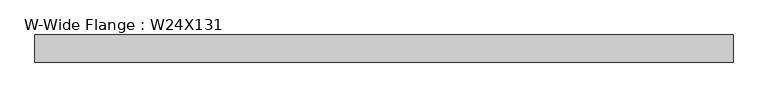
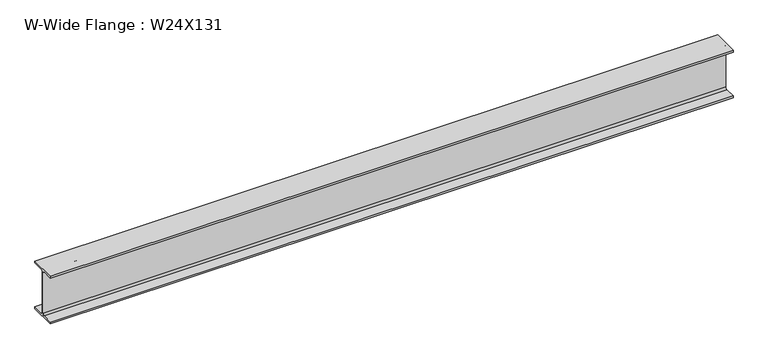
"""IFC4 building model written with IfcOpenShell, lengths in millimetres: beam geometry, W-Wide Flange : W24X131."""

from ifc_helpers import new_model, si_unit, point, frame, frame_2d, origin, place, context, project, spatial, polyline, circle_curve, trimmed, segment, composite_curve, outline, extrude, source, transform, mapped, element, save


def w_wide_flange_w24x131_18549e9f(model_context):
    return source(origin(), model_context, "Body", "SweptSolid", [
        extrude(outline(composite_curve([segment(polyline([(163.83, -286.766), (163.83, -311.15), (-163.83, -311.15), (-163.83, -286.766), (-30.9245, -286.766)]), True, "CONTINUOUS"), segment(trimmed(circle_curve(frame_2d((-30.9245, -263.525)), 23.241), [point((-30.9245, -286.766))], [point((-7.6835, -263.525))], True, "CARTESIAN"), True, "CONTINUOUS"), segment(polyline([(-7.6835, -263.525), (-7.6835, 263.525)]), True, "CONTINUOUS"), segment(trimmed(circle_curve(frame_2d((-30.9245, 263.525)), 23.241), [point((-7.6835, 263.525))], [point((-30.9245, 286.766))], True, "CARTESIAN"), True, "CONTINUOUS"), segment(polyline([(-30.9245, 286.766), (-163.83, 286.766), (-163.83, 311.15), (163.83, 311.15), (163.83, 286.766), (30.9245, 286.766)]), True, "CONTINUOUS"), segment(trimmed(circle_curve(frame_2d((30.9245, 263.525)), 23.241), [point((30.9245, 286.766))], [point((7.6835, 263.525))], True, "CARTESIAN"), True, "CONTINUOUS"), segment(polyline([(7.6835, 263.525), (7.6835, -263.525)]), True, "CONTINUOUS"), segment(trimmed(circle_curve(frame_2d((30.9245, -263.525)), 23.241), [point((7.6835, -263.525))], [point((30.9245, -286.766))], True, "CARTESIAN"), True, "CONTINUOUS"), segment(polyline([(30.9245, -286.766), (163.83, -286.766)]), True, "CONTINUOUS")], self_intersect=False)), frame((-4213.6230758, 0.0, 0.0), z_axis=(1.0, 0.0, 0.0), x_axis=(0.0, 1.0, 0.0)), (0.0, 0.0, 1.0), 8427.2461516),
    ])


if __name__ == "__main__":
    model = new_model("IFC4")
    model_context = context("Model", 3, world=origin())
    ifc_project = project(units=[si_unit("LENGTHUNIT", "METRE", prefix="MILLI")], contexts=[model_context])
    site = spatial("IfcSite", under=ifc_project)
    building = spatial("IfcBuilding", under=site)
    placement = place(None, origin())
    w_wide_flange_w24x131_shape = w_wide_flange_w24x131_18549e9f(model_context)
    element("IfcBeam", 1, ObjectType="W-Wide Flange : W24X131", at=placement, inside=building, context=model_context, shape_type="MappedRepresentation", body=[
        mapped(w_wide_flange_w24x131_shape, transform((0.0, 0.0, 0.0), x_axis=(1.0, 0.0, 0.0), y_axis=(0.0, 1.0, 0.0), z_axis=(0.0, 0.0, 1.0))),
    ])
    save(model, "model.ifc")

# Revit data of these elements
# Type "W-Wide Flange : W24X131"
#   Assembly Code = "B10"
#   W = 131
#   Start Extension Calculation [instance default] = 10' - 0"
#   Start Extension [instance default] = -0' - 0 1/2"
#   End Extension Calculation [instance default] = 10' - 0"
#   End Extension [instance default] = -0' - 0 1/2"
#   Length [instance default] = 5' - 0"
#   bf = 1' - 0.9"
#   d = 2' - 0 1/2"
#   k = 0' - 1 7/8"
#   k2 = 0' - 0.915"
#   tf = 0' - 0.96"
#   tw = 0' - 0.605"
#   A = 0.267361 SF
#   Beam Material [instance default] = Metal - Steel - ASTM A992
# Element 1 (IfcBeam, "W-Wide Flange : W24X131")
#   Materials on its faces: "Metal - Steel - ASTM A992"
# Materials
#   "Metal - Steel - ASTM A992": class "Metal", colour RGB 128 0 0, transparency 0
